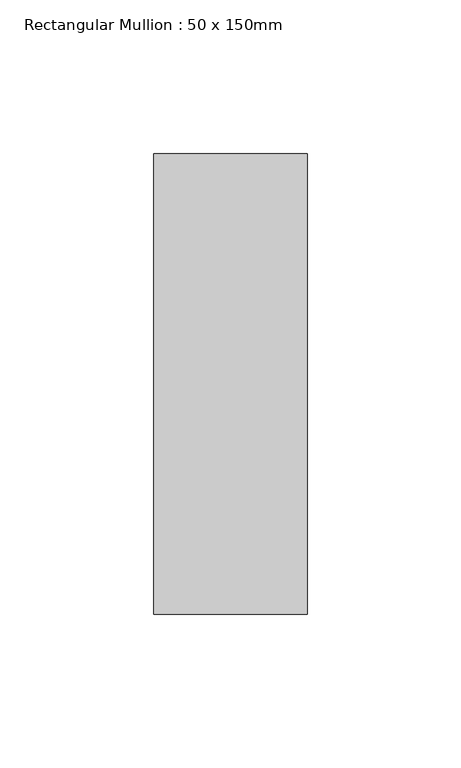
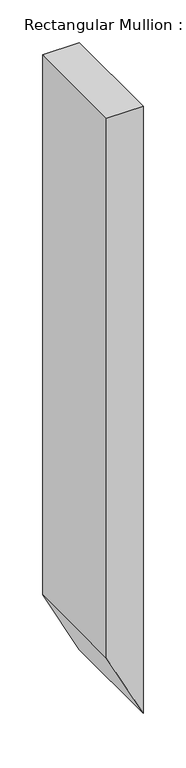
"""IFC4 building model written with IfcOpenShell, lengths in millimetres: member geometry, Rectangular Mullion : 50 x 150mm."""

from ifc_helpers import new_model, si_unit, frame, origin, place, context, project, spatial, polyline, outline, extrude, source, transform, mapped, element, save


def rectangular_mullion_50_x_150mm_83473cdf(model_context):
    return source(origin(), model_context, "Body", "SweptSolid", [
        extrude(outline(polyline([(0.0, 0.0), (0.0, -50.0), (-774.3867239, -50.0), (-870.4358302, 0.0), (0.0, 0.0)])), frame((0.0, -75.0, 0.0), z_axis=(0.0, 1.0, 0.0), x_axis=(0.0, 0.0, 1.0)), (0.0, 0.0, 1.0), 150.0),
    ])


if __name__ == "__main__":
    model = new_model("IFC4")
    model_context = context("Model", 3, world=origin())
    ifc_project = project(units=[si_unit("LENGTHUNIT", "METRE", prefix="MILLI")], contexts=[model_context])
    site = spatial("IfcSite", under=ifc_project)
    building = spatial("IfcBuilding", under=site)
    placement = place(None, origin())
    rectangular_mullion_50_x_150mm_shape = rectangular_mullion_50_x_150mm_83473cdf(model_context)
    element("IfcMember", 1, ObjectType="Rectangular Mullion : 50 x 150mm", at=placement, inside=building, context=model_context, shape_type="MappedRepresentation", body=[
        mapped(rectangular_mullion_50_x_150mm_shape, transform((0.0, 0.0, 0.0), x_axis=(1.0, 0.0, 0.0), y_axis=(0.0, 1.0, 0.0), z_axis=(0.0, 0.0, 1.0))),
    ])
    save(model, "model.ifc")

# Revit data of these elements
# Type "Rectangular Mullion : 50 x 150mm"
#   built-in parameter 1007304 = 0.492126 (stored number, unit not read)
#   built-in parameter 1007301 = 0.082021 (stored number, unit not read)
#   built-in parameter 1007300 = 0.082021 (stored number, unit not read)
# Element 1 (IfcMember, "Rectangular Mullion : 50 x 150mm")
#   Materials on its faces: "Aluminium"
# Materials
#   "Aluminium": class "Metal", colour RGB 247 247 247, transparency 0, Description = "Aluminium 6061", Cost = 0
